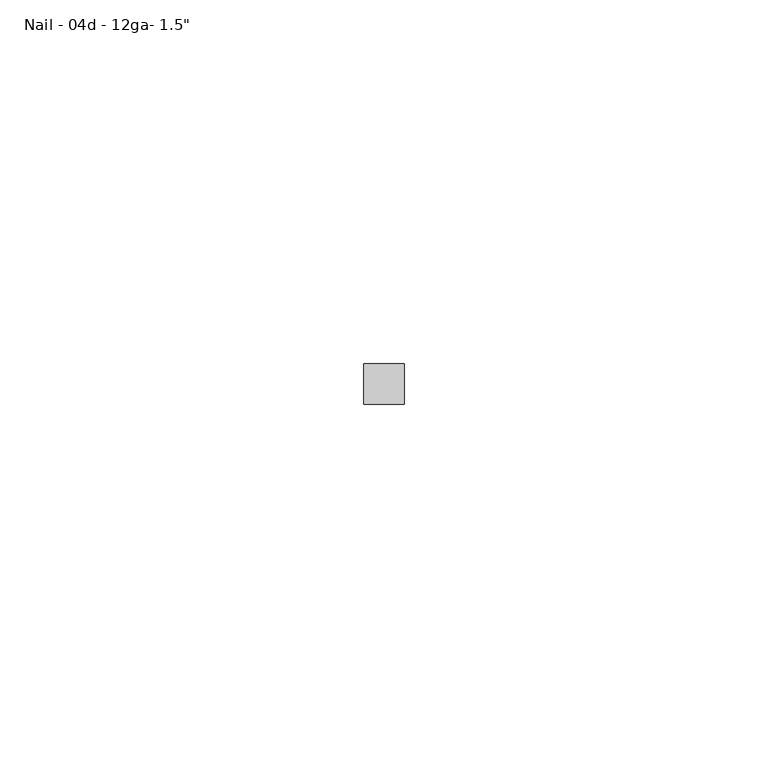
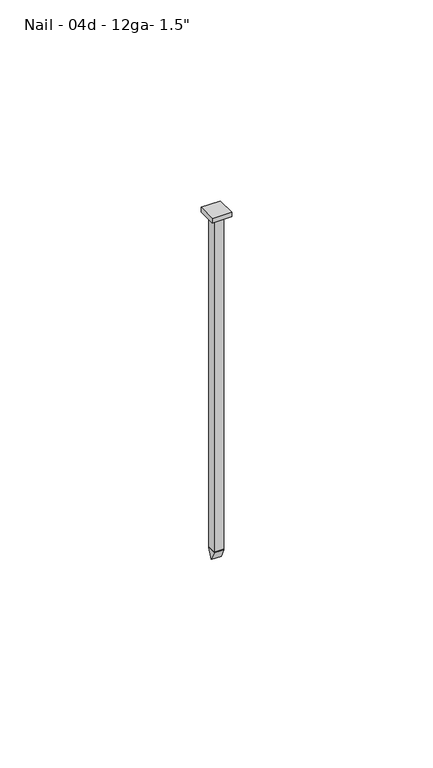
"""IFC4 building model written with IfcOpenShell, lengths in millimetres: fastener geometry."""

from ifc_helpers import new_model, si_unit, frame, origin, origin_with_axes, place, context, project, spatial, polyline, outline, extrude, source, transform, mapped, element, save


def fastener_92d45581(model_context):
    return source(origin(), model_context, "Body", "SweptSolid", [
        extrude(outline(polyline([(0.0, -104.3686), (-1.3843, -101.6), (1.3843, -101.6), (0.0, -104.3686)])), frame((-1.3843, 0.0, 0.0), z_axis=(1.0, 0.0, 0.0), x_axis=(0.0, 1.0, 0.0)), (0.0, 0.0, 1.0), 2.7686),
        extrude(outline(polyline([(-2.7686, -2.7686), (-2.7686, 2.7686), (2.7686, 2.7686), (2.7686, -2.7686), (-2.7686, -2.7686)])), origin_with_axes(), (0.0, 0.0, 1.0), 1.3843),
        extrude(outline(polyline([(-1.3843, 1.3843), (1.3843, 1.3843), (1.3843, -1.3843), (-1.3843, -1.3843), (-1.3843, 1.3843)])), frame((0.0, 0.0, -101.6), z_axis=(0.0, 0.0, 1.0), x_axis=(1.0, 0.0, 0.0)), (0.0, 0.0, 1.0), 101.6),
    ])


if __name__ == "__main__":
    model = new_model("IFC4")
    model_context = context("Model", 3, world=origin())
    ifc_project = project(units=[si_unit("LENGTHUNIT", "METRE", prefix="MILLI")], contexts=[model_context])
    site = spatial("IfcSite", under=ifc_project)
    building = spatial("IfcBuilding", under=site)
    placement = place(None, origin())
    fastener_shape = fastener_92d45581(model_context)
    element("IfcFastener", 1, ObjectType="060523 - W_P_C - Fastenings - Generic - SQUARE : Nail - 04d - 12ga- 1.5\"", at=placement, inside=building, context=model_context, shape_type="MappedRepresentation", body=[
        mapped(fastener_shape, transform((0.0, 0.0, 0.0), x_axis=(1.0, 0.0, 0.0), y_axis=(0.0, 1.0, 0.0), z_axis=(0.0, 0.0, 1.0))),
    ])
    save(model, "model.ifc")

# Revit data of these elements
# Type "060523 - W_P_C - Fastenings - Generic - SQUARE : Nail - 04d - 12ga- 1.5\""
#   Washer_Thickness = 0' - 0.00333"
#   Washer Radius = 0' - 0.0645"
#   Washer Offset - Head = 0' - 0"
#   Washer Offset = 0' - 0"
#   Thickness_of_Substrate [instance default] = 0' - 1"
#   Side = 0' - 0 37/64"
#   Radius = 0' - 0.0545"
#   Length [instance default] = 0' - 1 1/2"
#   Head Size = 0' - 1"
#   Head Radius = 0' - 0 1/2"
#   Head Height = 0' - 0.01"
#   Double Diameter = 0' - 0.218"
#   Diameter = 0' - 0.109"
#   Default Elevation = 4' - 0"
#   Washer_Nut_Visibility = no
#   Washer_Head_Visibility = no
#   Round_Head_Visibility = yes
#   Point Visibility = yes
#   Nut_Visibility = no
#   Hex_Head_Visiblilty = no
#   Washer Material = none
#   Bolt Material (Size) = AT SILL - FASTENER AT 24" O.C.
# Element 1 (IfcFastener, "060523 - W_P_C - Fastenings - Generic - SQUARE : Nail - 04d - 12ga- 1.5\"")
#   Length = 0' - 4"
# Materials
#   "AT SILL - FASTENER AT 24\" O.C.": class "Generic", colour RGB 120 120 120, transparency 0, Cost = 0
